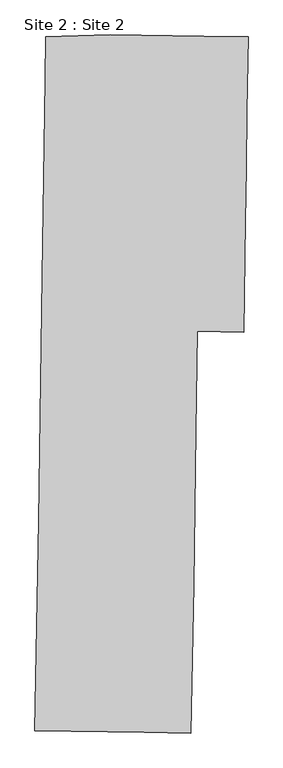
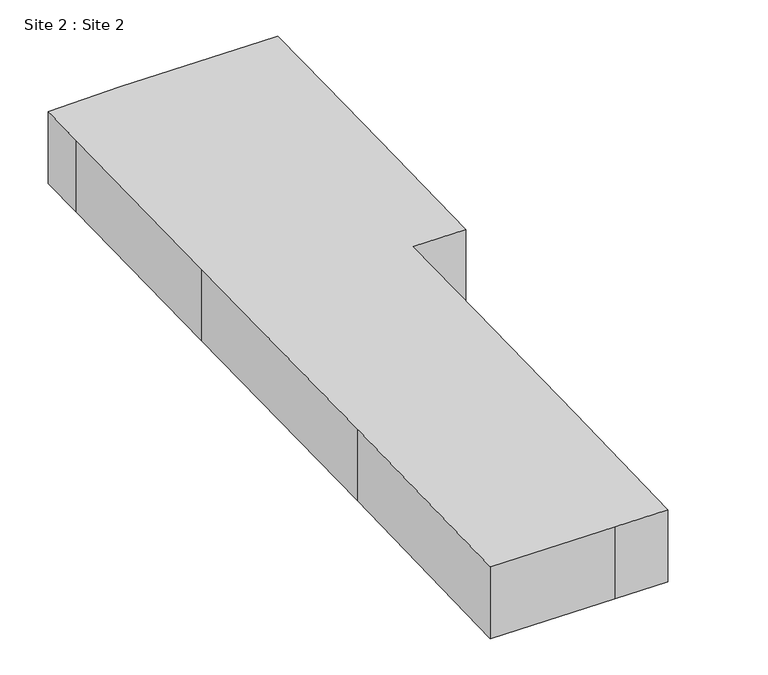
"""IFC4 building model written with IfcOpenShell, lengths in millimetres: geographic element geometry, Site 2 : Site 2."""

from ifc_helpers import new_model, si_unit, frame, origin, place, context, project, spatial, polyline, outline, extrude, source, transform, mapped, element, save


def site_2_site_2_3b6e2255(model_context):
    return source(origin(), model_context, "Body", "SweptSolid", [
        extrude(outline(polyline([(120717.2731903, 172767.4272861), (122241.1139378, 172745.35103), (122118.9607555, 164313.5772706), (122024.7702095, 157811.9588991), (121937.9388652, 151818.3184839), (121755.444644, 139221.4302436), (116472.7998231, 139297.9612197), (116309.4385452, 128021.7479412), (116054.8295435, 110447.0482146), (115710.4035382, 93686.5596005), (110427.7587173, 93763.0905766), (98033.8584853, 93942.6440605), (98481.3053429, 117814.2738003), (98883.0867278, 145547.7284229), (99206.8664614, 167897.0230564), (99277.508911, 172773.2050891), (106596.3537265, 172972.0005228), (120717.2731903, 172767.4272861)])), frame((0.0, 0.0, 266395.2), z_axis=(0.0, 0.0, 1.0), x_axis=(1.0, 0.0, 0.0)), (0.0, 0.0, 1.0), 7620.0),
    ])


if __name__ == "__main__":
    model = new_model("IFC4")
    model_context = context("Model", 3, world=origin())
    ifc_project = project(units=[si_unit("LENGTHUNIT", "METRE", prefix="MILLI")], contexts=[model_context])
    site = spatial("IfcSite", under=ifc_project)
    building = spatial("IfcBuilding", under=site)
    placement = place(None, origin())
    site_2_site_2_shape = site_2_site_2_3b6e2255(model_context)
    element("IfcGeographicElement", 1, ObjectType="Site 2 : Site 2", at=placement, inside=building, context=model_context, shape_type="MappedRepresentation", body=[
        mapped(site_2_site_2_shape, transform((0.0, 0.0, 0.0), x_axis=(1.0, 0.0, 0.0), y_axis=(0.0, 1.0, 0.0), z_axis=(0.0, 0.0, 1.0))),
    ])
    save(model, "model.ifc")

# Revit data of these elements
# Element 1 (IfcGeographicElement, "Site 2 : Site 2")
#   Materials on its faces: "EXISTING BUILDING"
# Materials
#   "EXISTING BUILDING": class "Generic", colour RGB 120 120 120, transparency 0, Cost = 0
